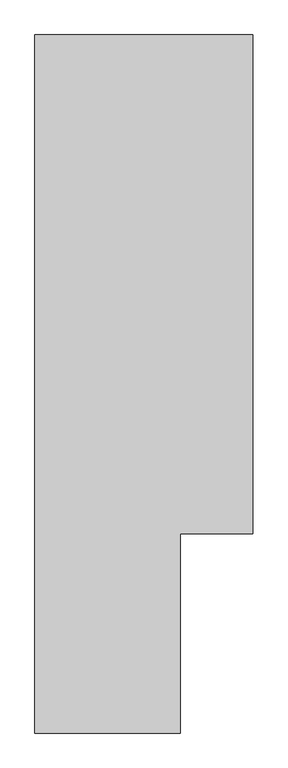
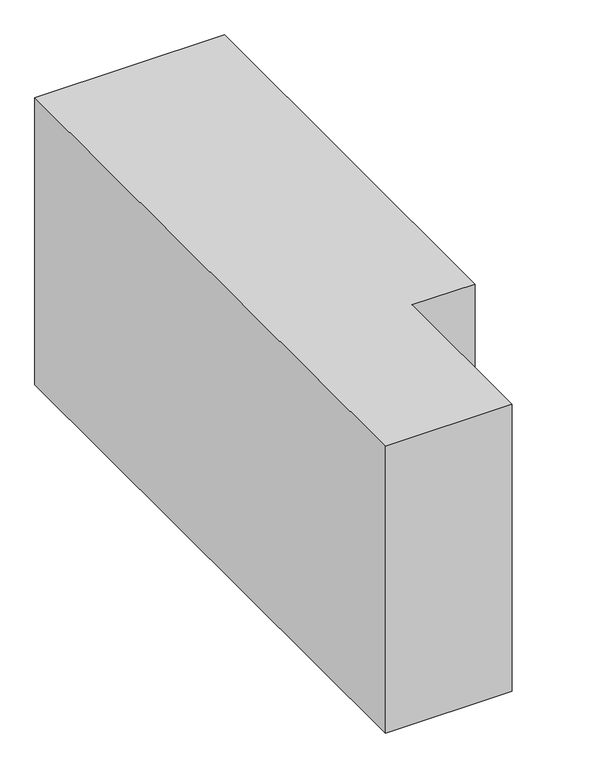
"""IFC4 building model written with IfcOpenShell, lengths in millimetres: proxy geometry, 0_3d."""

from ifc_helpers import new_model, si_unit, origin, origin_with_axes, place, context, project, spatial, polyline, outline, extrude, source, transform, mapped, element, save


def generic_models_c9c81b52(model_context):
    return source(origin(), model_context, "Body", "SweptSolid", [
        extrude(outline(polyline([(0.0, 0.0), (0.0, 5772.0), (1802.0709768, 5772.0), (1802.0709768, 1646.0204176), (1202.0709768, 1646.0204176), (1202.0709768, 0.0), (0.0, 0.0)])), origin_with_axes(), (0.0, 0.0, 1.0), 2880.0),
    ])


if __name__ == "__main__":
    model = new_model("IFC4")
    model_context = context("Model", 3, world=origin())
    ifc_project = project(units=[si_unit("LENGTHUNIT", "METRE", prefix="MILLI")], contexts=[model_context])
    site = spatial("IfcSite", under=ifc_project)
    building = spatial("IfcBuilding", under=site)
    placement = place(None, origin())
    generic_models_shape = generic_models_c9c81b52(model_context)
    element("IfcBuildingElementProxy", 1, Name="0_3d", ObjectType="0_3d", at=placement, inside=building, context=model_context, shape_type="MappedRepresentation", body=[
        mapped(generic_models_shape, transform((0.0, 0.0, 0.0), x_axis=(1.0, 0.0, 0.0), y_axis=(0.0, 1.0, 0.0), z_axis=(0.0, 0.0, 1.0))),
    ])
    save(model, "model.ifc")

# Revit data of these elements
# Element 1 (IfcBuildingElementProxy, "0_3d")
#   Materials on its faces: "*1"
# Materials
#   "*1": class "Unassigned", colour RGB 175 175 175, transparency 0
